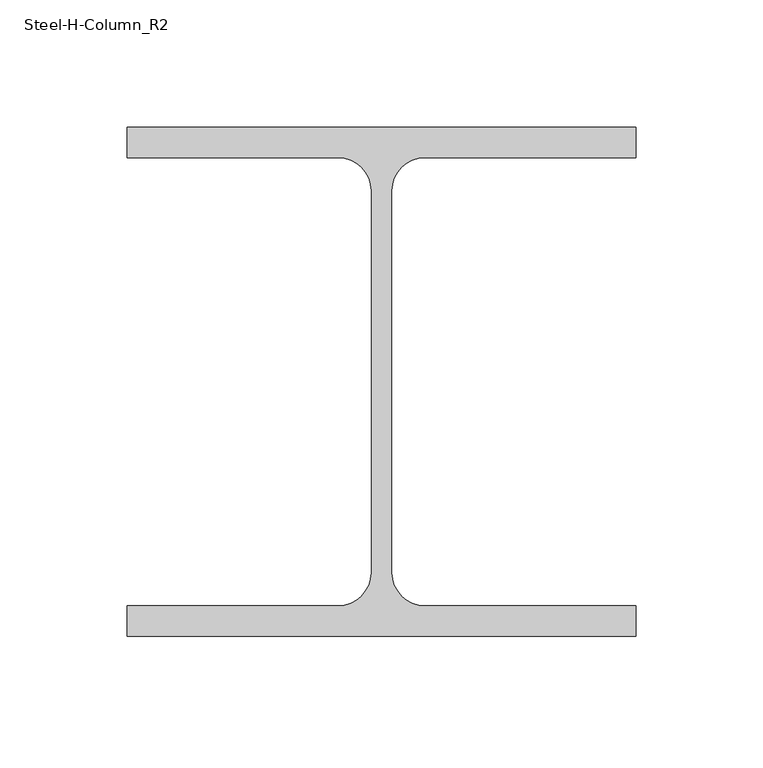
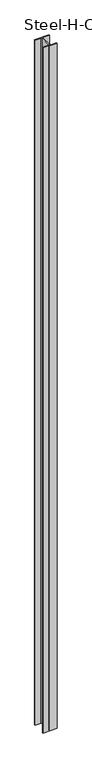
"""IFC4 building model written with IfcOpenShell, lengths in millimetres: column geometry, Steel-H-Column_R2 : CL121_H-200×200x8x12_C2."""

from ifc_helpers import new_model, si_unit, point, frame, frame_2d, origin, place, context, project, spatial, polyline, circle_curve, trimmed, segment, composite_curve, outline, extrude, source, transform, mapped, element, save


def steel_h_column_r2_bdd731d0(model_context):
    return source(origin(), model_context, "Body", "SweptSolid", [
        extrude(outline(composite_curve([segment(polyline([(100.0, 100.0), (100.0, 88.0), (17.0, 88.0)]), True, "CONTINUOUS"), segment(trimmed(circle_curve(frame_2d((17.0, 75.0)), 13.0), [point((17.0, 88.0))], [point((4.0, 75.0))], True, "CARTESIAN"), True, "CONTINUOUS"), segment(polyline([(4.0, 75.0), (4.0, -75.0)]), True, "CONTINUOUS"), segment(trimmed(circle_curve(frame_2d((17.0, -75.0)), 13.0), [point((4.0, -75.0))], [point((17.0, -88.0))], True, "CARTESIAN"), True, "CONTINUOUS"), segment(polyline([(17.0, -88.0), (100.0, -88.0), (100.0, -100.0), (-100.0, -100.0), (-100.0, -88.0), (-17.0, -88.0)]), True, "CONTINUOUS"), segment(trimmed(circle_curve(frame_2d((-17.0, -75.0)), 13.0), [point((-17.0, -88.0))], [point((-4.0, -75.0))], True, "CARTESIAN"), True, "CONTINUOUS"), segment(polyline([(-4.0, -75.0), (-4.0, 75.0)]), True, "CONTINUOUS"), segment(trimmed(circle_curve(frame_2d((-17.0, 75.0)), 13.0), [point((-4.0, 75.0))], [point((-17.0, 88.0))], True, "CARTESIAN"), True, "CONTINUOUS"), segment(polyline([(-17.0, 88.0), (-100.0, 88.0), (-100.0, 100.0), (100.0, 100.0)]), True, "CONTINUOUS")], self_intersect=False)), frame((0.0, 0.0, 50.0), z_axis=(0.0, 0.0, 1.0), x_axis=(1.0, 0.0, 0.0)), (0.0, 0.0, 1.0), 10150.0),
    ])


if __name__ == "__main__":
    model = new_model("IFC4")
    model_context = context("Model", 3, world=origin())
    ifc_project = project(units=[si_unit("LENGTHUNIT", "METRE", prefix="MILLI")], contexts=[model_context])
    site = spatial("IfcSite", under=ifc_project)
    building = spatial("IfcBuilding", under=site)
    placement = place(None, origin())
    steel_h_column_r2_shape = steel_h_column_r2_bdd731d0(model_context)
    element("IfcColumn", 1, ObjectType="Steel-H-Column_R2 : CL121_H-200×200x8x12_C2", at=placement, inside=building, context=model_context, shape_type="MappedRepresentation", body=[
        mapped(steel_h_column_r2_shape, transform((0.0, 0.0, 0.0), x_axis=(1.0, 0.0, 0.0), y_axis=(0.0, 1.0, 0.0), z_axis=(0.0, 0.0, 1.0))),
    ])
    save(model, "model.ifc")

# Revit data of these elements
# Type "Steel-H-Column_R2 : CL121_H-200×200x8x12_C2"
#   SteelWeight = "Medium"
#   Surface Area = 1.16168 m²/m
#   Section Area = 63.5307 cm²
#   Mass per Unit Length = 49.8716 kg/m
#   B = 200 mm
#   H = 200 mm
#   r = 13 mm
#   tw = 8 mm
#   tf = 12 mm
#   hec_material4 [instance default] = none
#   hec_material2 [instance default] = none
#   hec_material1 [instance default] = none
#   hec_material3 [instance default] = none
#   Structural Material [instance default] = Steel, 45-345
#   Assembly Code = ""
# Element 1 (IfcColumn, "Steel-H-Column_R2 : CL121_H-200×200x8x12_C2")
#   Materials on its faces: "Steel, 45-345"
# Materials
#   "Steel, 45-345": class "Metal", colour RGB 189 187 185, transparency 0, Description = "Steel 345 MPa", Cost = 0
